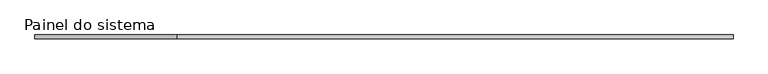
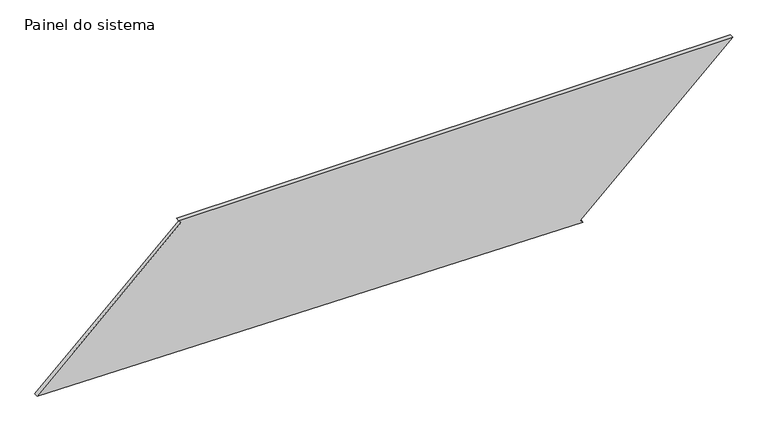
"""IFC4 building model written with IfcOpenShell, lengths in millimetres: plate geometry, Painel do sistema : Envidraçado."""

from ifc_helpers import new_model, si_unit, frame, origin, place, context, project, spatial, polyline, outline, extrude, source, transform, mapped, element, save


def painel_do_sistema_2618dfdb(model_context):
    return source(origin(), model_context, "Body", "SweptSolid", [
        extrude(outline(polyline([(0.0, 1343.8693502), (18.3764951, 1326.9192934), (970.8719484, 2359.5723533), (970.8719484, -1397.9798524), (952.4954533, -1381.0297955), (49.9102838, -2359.5723533), (0.0, 1343.8693502)])), frame((0.0, 24.5, 0.0), z_axis=(0.0, 1.0, 0.0), x_axis=(0.0, 0.0, 1.0)), (0.0, 0.0, 1.0), 25.0),
    ])


if __name__ == "__main__":
    model = new_model("IFC4")
    model_context = context("Model", 3, world=origin())
    ifc_project = project(units=[si_unit("LENGTHUNIT", "METRE", prefix="MILLI")], contexts=[model_context])
    site = spatial("IfcSite", under=ifc_project)
    building = spatial("IfcBuilding", under=site)
    placement = place(None, origin())
    painel_do_sistema_shape = painel_do_sistema_2618dfdb(model_context)
    element("IfcPlate", 1, ObjectType="Painel do sistema : Envidraçado", at=placement, inside=building, context=model_context, shape_type="MappedRepresentation", body=[
        mapped(painel_do_sistema_shape, transform((0.0, 0.0, 0.0), x_axis=(1.0, 0.0, 0.0), y_axis=(0.0, 1.0, 0.0), z_axis=(0.0, 0.0, 1.0))),
    ])
    save(model, "model.ifc")

# Revit data of these elements
# Type "Painel do sistema : Envidraçado"
#   Construction Type Id = "GSP4R"
#   Analytic Construction = "Vidraça única Pilkington 1/8 pol"
#   Visual Light Transmittance = 0.9
#   Solar Heat Gain Coefficient = 0.86
#   Heat Transfer Coefficient (U) = 6.7069 W/(m²·K)
# Element 1 (IfcPlate, "Painel do sistema : Envidraçado")
#   Materials on its faces: "Vidro"
# Materials
#   "Vidro": class "Vidro", colour RGB 0 128 192, transparency 0.9, Description = "Vidro de sílica", Cost = 0
